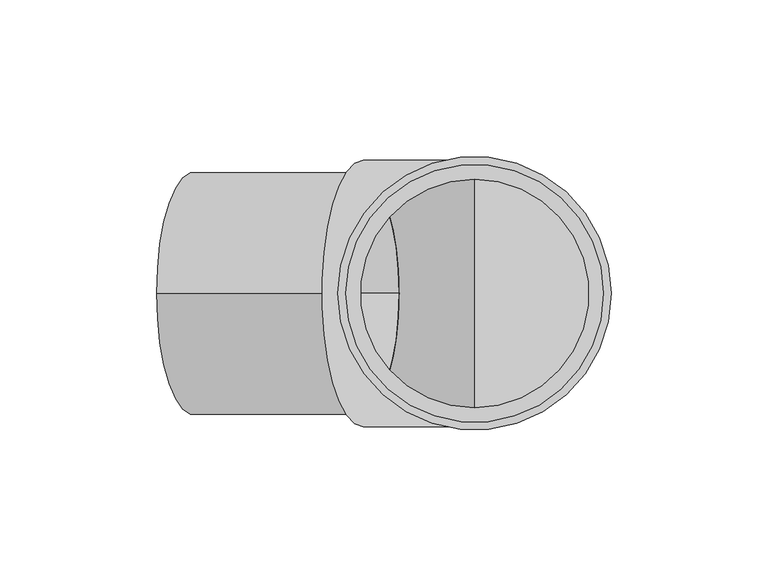
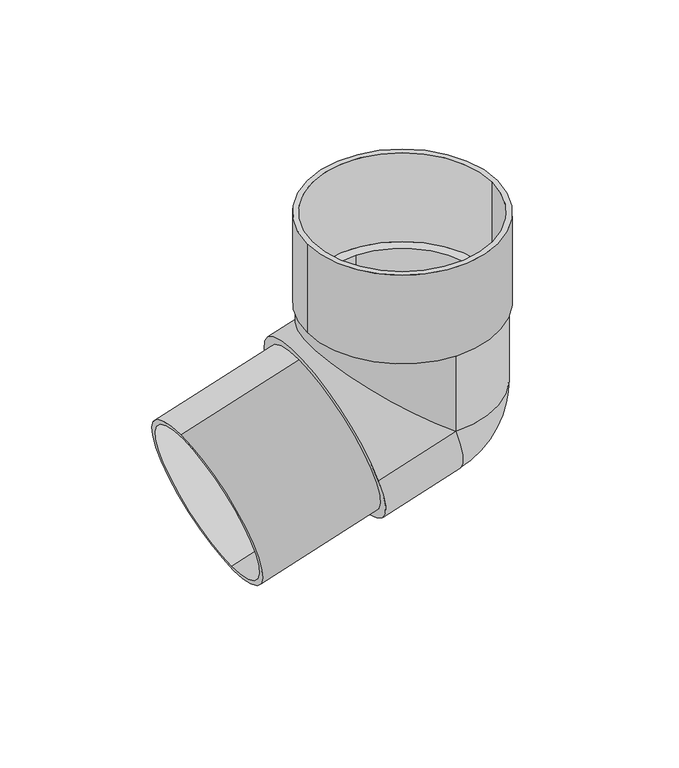
"""IFC4 building model written with IfcOpenShell, lengths in millimetres: proxy geometry, ⇲ Колено трубы 108 : ⇲ Колено трубы 108."""

from ifc_helpers import new_model, si_unit, point, frame, origin, origin_with_axes, origin_2d, place, context, project, spatial, polyline, circle_curve, ellipse_curve, trimmed, segment, composite_curve, outline, extrude, source, transform, mapped, element, save
from ifc_brep_helpers import plane_surface, cylinder_surface, revolved_surface, advanced_brep


def generic_models_5036811a(model_context):
    return source(origin(), model_context, "Body", "SolidModel", [
        extrude(outline(composite_curve([segment(trimmed(circle_curve(origin_2d(), 38.8), [point((0.0, -38.8))], [point((0.0, 38.8000001))], False, "CARTESIAN"), True, "CONTINUOUS"), segment(trimmed(circle_curve(origin_2d(), 38.8), [point((0.0, 38.8000001))], [point((0.0, -38.8))], False, "CARTESIAN"), True, "CONTINUOUS")], self_intersect=False), holes=[composite_curve([segment(trimmed(circle_curve(origin_2d(), 36.5), [point((0.0, -36.5))], [point((0.0, 36.5000001))], True, "CARTESIAN"), True, "CONTINUOUS"), segment(trimmed(circle_curve(origin_2d(), 36.5), [point((0.0, 36.5000001))], [point((0.0, -36.5))], True, "CARTESIAN"), True, "CONTINUOUS")], self_intersect=False)]), frame((-89.3993125, 0.0, -109.2975975), z_axis=(0.9510565162951546, 0.0, 0.30901699437494445), x_axis=(0.0, 1.0, 0.0)), (0.0, 0.0, 1.0), 56.7),
        advanced_brep(
        [(41.1, 0.0, -43.0), (-41.1, 0.0, -43.0), (0.0, -36.41, -43.0), (0.0, 36.41, -43.0), (0.0, -42.5, -43.0), (0.0, 42.5, -43.0), (0.0, 42.5, -80.25), (0.0, -42.5, -80.25), (42.5, 0.0, -80.25), (0.0, 36.41, -80.25), (0.0, -36.41, -80.25), (-35.4744081, -42.5, -91.7763339), (-35.4744081, 42.5, -91.7763339), (-35.4744081, -36.41, -91.7763339), (-35.4744081, 36.41, -91.7763339), (13.1332223, 0.0, -120.6699019), (-43.6, 0.0, 0.0), (43.6, 0.0, 0.0), (-41.1, 0.0, 0.0), (41.1, 0.0, 0.0), (-43.6, 0.0, -43.0), (43.6, 0.0, -43.0)],
        [
            (0, 1, circle_curve(frame((0.0, 0.0, -43.0), z_axis=(0.0, 0.0, 1.0), x_axis=(1.0, 0.0, 0.0)), 41.1)),
            (1, 0, circle_curve(frame((0.0, 0.0, -43.0), z_axis=(0.0, 0.0, 1.0), x_axis=(1.0, 0.0, 0.0)), 41.1)),
            (2, 3, circle_curve(frame((0.0, 0.0, -43.0), z_axis=(0.0, 0.0, -1.0), x_axis=(0.0, 1.0, 0.0)), 36.41)),
            (3, 2, circle_curve(frame((0.0, 0.0, -43.0), z_axis=(0.0, 0.0, -1.0), x_axis=(0.0, 1.0, 0.0)), 36.41)),
            (4, 5, circle_curve(frame((0.0, 0.0, -43.0), z_axis=(0.0, 0.0, -1.0), x_axis=(0.0, 1.0, 0.0)), 42.5)),
            (5, 6),
            (6, 7, ellipse_curve(frame((0.0, 0.0, -80.25), z_axis=(0.5877852522924751, 0.0, 0.8090169943749459), x_axis=(-0.8090169943749458, 0.0, 0.5877852522924751)), 52.532889, 42.5)),
            (7, 4),
            (7, 8, circle_curve(frame((0.0, 0.0, -80.25), z_axis=(0.0, 0.0, 1.0), x_axis=(0.0, 1.0, 0.0)), 42.5)),
            (8, 6, circle_curve(frame((0.0, 0.0, -80.25), z_axis=(0.0, 0.0, 1.0), x_axis=(0.0, 1.0, 0.0)), 42.5)),
            (5, 4, circle_curve(frame((0.0, 0.0, -43.0), z_axis=(0.0, 0.0, -1.0), x_axis=(0.0, 1.0, 0.0)), 42.5)),
            (3, 9),
            (9, 10, circle_curve(frame((0.0, 0.0, -80.25), z_axis=(0.0, 0.0, -1.0), x_axis=(0.0, 1.0, 0.0)), 36.41)),
            (10, 2),
            (10, 9, ellipse_curve(frame((0.0, 0.0, -80.25), z_axis=(-0.5877852522924751, 0.0, -0.8090169943749459), x_axis=(0.8090169943749458, 0.0, -0.5877852522924751)), 45.0052351, 36.41)),
            (11, 12, circle_curve(frame((-35.4744081, 0.0, -91.7763339), z_axis=(-0.9510565162951546, 0.0, -0.30901699437494445), x_axis=(0.0, 1.0, 0.0)), 42.5)),
            (12, 11, circle_curve(frame((-35.4744081, 0.0, -91.7763339), z_axis=(-0.9510565162951546, 0.0, -0.30901699437494445), x_axis=(0.0, 1.0, 0.0)), 42.5)),
            (13, 14, circle_curve(frame((-35.4744081, 0.0, -91.7763339), z_axis=(0.9510565162951546, 0.0, 0.30901699437494445), x_axis=(0.0, 1.0, 0.0)), 36.41)),
            (14, 13, circle_curve(frame((-35.4744081, 0.0, -91.7763339), z_axis=(0.9510565162951546, 0.0, 0.30901699437494445), x_axis=(0.0, 1.0, 0.0)), 36.41)),
            (6, 12),
            (11, 7),
            (6, 15, circle_curve(frame((0.0, 0.0, -80.25), z_axis=(-0.9510565162951546, 0.0, -0.30901699437494445), x_axis=(0.0, 1.0, 0.0)), 42.5)),
            (15, 7, circle_curve(frame((0.0, 0.0, -80.25), z_axis=(-0.9510565162951546, 0.0, -0.30901699437494445), x_axis=(0.0, 1.0, 0.0)), 42.5)),
            (13, 10),
            (10, 9, circle_curve(frame((0.0, 0.0, -80.25), z_axis=(0.9510565162951546, 0.0, 0.30901699437494445), x_axis=(0.0, 1.0, 0.0)), 36.41)),
            (9, 14),
            (9, 10),
            (16, 17, circle_curve(origin_with_axes(), 43.6)),
            (17, 16, circle_curve(origin_with_axes(), 43.6)),
            (18, 19, circle_curve(frame((0.0, 0.0, 0.0), z_axis=(0.0, 0.0, -1.0), x_axis=(1.0, 0.0, 0.0)), 41.1)),
            (19, 18, circle_curve(frame((0.0, 0.0, 0.0), z_axis=(0.0, 0.0, -1.0), x_axis=(1.0, 0.0, 0.0)), 41.1)),
            (20, 21, circle_curve(frame((0.0, 0.0, -43.0), z_axis=(0.0, 0.0, -1.0), x_axis=(1.0, 0.0, 0.0)), 43.6)),
            (21, 20, circle_curve(frame((0.0, 0.0, -43.0), z_axis=(0.0, 0.0, -1.0), x_axis=(1.0, 0.0, 0.0)), 43.6)),
            (19, 0),
            (1, 18),
            (17, 21),
            (20, 16),
        ],
        [
            plane_surface(frame((0.0, 0.0, -43.0), z_axis=(0.0, 0.0, 1.0), x_axis=(0.0, 1.0, 0.0))),
            cylinder_surface(frame((0.0, 0.0, -43.0), z_axis=(0.0, 0.0, 1.0), x_axis=(0.0, 1.0, 0.0)), 42.5),
            revolved_surface(polyline([(0.0, 36.41, -80.25), (0.0, 36.41, -43.0)]), (0.0, 0.0, -43.0), (0.0, 0.0, -1.0)),
            revolved_surface(polyline([(0.0, 36.41, -106.70341346773566), (0.0, 36.41, -43.0)]), (0.0, 0.0, -43.0), (0.0, 0.0, -1.0)),
            plane_surface(frame((-35.4744081, 0.0, -91.7763339), z_axis=(-0.9510565162951546, 0.0, -0.30901699437494445), x_axis=(0.0, 1.0, 0.0))),
            cylinder_surface(frame((0.0, 0.0, -80.25), z_axis=(0.9510565162951546, 0.0, 0.30901699437494445), x_axis=(0.0, 1.0, 0.0)), 42.5),
            revolved_surface(polyline([(-35.47440809885558, 36.41, -91.77633390352219), (0.0, 36.41, -80.25)]), (0.0, 0.0, -80.25), (-0.9510565162951546, 0.0, -0.30901699437494445)),
            revolved_surface(polyline([(-35.47440809885558, 36.41, -91.77633390352219), (25.15869125673993, 36.41, -72.07544567924268)]), (0.0, 0.0, -80.25), (-0.9510565162951546, 0.0, -0.30901699437494445)),
            plane_surface(frame((0.0, -50.0, -80.25), z_axis=(0.0, 0.0, 1.0), x_axis=(1.0, 0.0, 0.0))),
            plane_surface(frame((0.0, -50.0, -80.25), z_axis=(-0.9510565162951546, 0.0, -0.30901699437494445), x_axis=(0.30901699437494445, 0.0, -0.9510565162951546))),
            revolved_surface(trimmed(ellipse_curve(frame((0.0, 0.0, -80.25), z_axis=(0.0, 0.0, -1.0), x_axis=(1.0, 0.0, 0.0)), 42.5, 42.5), [point((0.0, 42.5, -80.25))], [point((0.0, -42.5, -80.25))], True, "CARTESIAN"), (0.0, -50.0, -80.25), (0.0, -1.0, 0.0)),
            plane_surface(frame((41.1, 0.0, 0.0), z_axis=(0.0, 0.0, 1.0), x_axis=(0.0, 1.0, 0.0))),
            plane_surface(frame((41.1, 0.0, -43.0), z_axis=(0.0, 0.0, -1.0), x_axis=(0.0, -1.0, 0.0))),
            revolved_surface(polyline([(41.1, 0.0, -43.0), (41.1, 0.0, 0.0)]), (0.0, 0.0, -43.0), (0.0, 0.0, -1.0)),
            cylinder_surface(origin_with_axes(), 43.6),
        ],
        [
            (0, [[1, 2], [3, 4]]),
            (1, [[5, 6, 7, 8]]),
            (1, [[9, 10, -6, 11, -8]]),
            (2, [[12, 13, 14, -4]]),
            (3, [[-14, 15, -12, -3]]),
            (4, [[16, 17], [18, 19]]),
            (5, [[20, -16, 21, -7]]),
            (5, [[-20, 22, 23, -21, -17]]),
            (6, [[24, 25, 26, -18]]),
            (7, [[-24, -19, -26, -15]]),
            (8, [[-13, 27]]),
            (9, [[-25, -27]]),
            (10, [[-23, -22, -10, -9]]),
            (11, [[28, 29], [30, 31]]),
            (12, [[32, 33], [-11, -5]]),
            (13, [[34, -2, 35, -31]]),
            (13, [[-35, -1, -34, -30]]),
            (14, [[36, -32, 37, -29]]),
            (14, [[-37, -33, -36, -28]]),
        ],
    ),
    ])


if __name__ == "__main__":
    model = new_model("IFC4")
    model_context = context("Model", 3, world=origin())
    ifc_project = project(units=[si_unit("LENGTHUNIT", "METRE", prefix="MILLI")], contexts=[model_context])
    site = spatial("IfcSite", under=ifc_project)
    building = spatial("IfcBuilding", under=site)
    placement = place(None, origin())
    generic_models_shape = generic_models_5036811a(model_context)
    element("IfcBuildingElementProxy", 1, Name="⇲ Колено трубы 108 : ⇲ Колено трубы 108", ObjectType="⇲ Колено трубы 108 : ⇲ Колено трубы 108", at=placement, inside=building, context=model_context, shape_type="MappedRepresentation", body=[
        mapped(generic_models_shape, transform((0.0, 0.0, 0.0), x_axis=(1.0, 0.0, 0.0), y_axis=(0.0, 1.0, 0.0), z_axis=(0.0, 0.0, 1.0))),
    ])
    save(model, "model.ifc")

# Revit data of these elements
# Type "⇲ Колено трубы 108 : ⇲ Колено трубы 108"
#   Description = "Предназначено для изменения направления стока по трубе. Также применяется для обхода архитектурных элементов\r\nфасада"
#   Manufacturer = "ТехноНИКОЛЬ"
#   Model = "Комплектующие к водосточным системам"
#   URL = "https://tn-vodostok.ru/catalog/pvh/"
#   ADSK_Обозначение = "ТехноНИКОЛЬ"
#   ADSK_Наименование краткое = "Колено 108°"
#   ADSK_Наименование = "Колено трубы 108°"
#   ADSK_Масса_Текст = ""
#   ADSK_Марка = ""
#   ADSK_Код изделия = ""
#   ADSK_Завод-изготовитель = "ТехноНИКОЛЬ"
#   ADSK_Единица измерения = "шт."
#   ADSK_Группирование = "Комплектующие к водосточным системам"
#   ADSK_URL страницы изделия = "https://tn-vodostok.ru/catalog/pvh/"
#   ADSK_URL документации изделия = "https://tn-vodostok.ru/upload/iblock/c42/c427963cb77eb5c3c51f0cfb870e9e52.pdf"
#   Угол поворота хомута [instance default] = 0.00°
#   ADSK_Размер_Ширина = 145.3 mm
#   ADSK_Размер_Диаметр = 82.2 mm
#   ADSK_Размер_Высота = 160.5 mm
#   ADSK_Количество = 1
#   ADSK_Материал [instance default] = TN_Пластик_Коричневый_RAL8019
#   Default Elevation = 0
# Element 1 (IfcBuildingElementProxy, "⇲ Колено трубы 108 : ⇲ Колено трубы 108")
#   Materials on its faces: "TN_Пластик_Коричневый_RAL8019"
# Materials
#   "TN_Пластик_Коричневый_RAL8019": class "Типовые", colour RGB 61 54 53, transparency 0, Cost = 0
